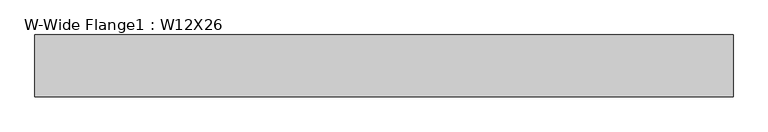
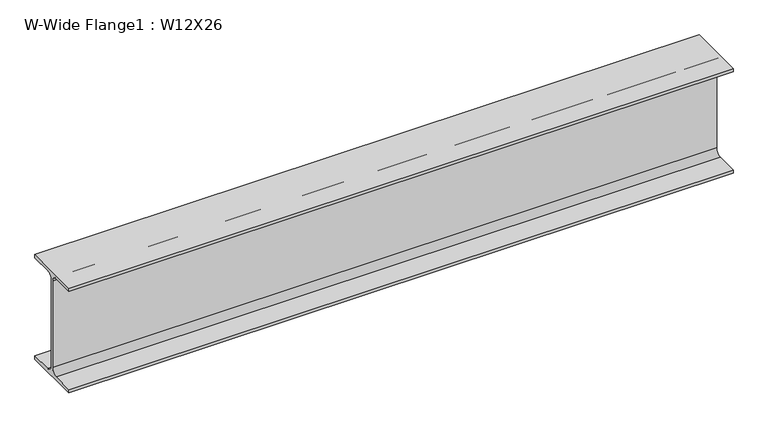
"""IFC4 building model written with IfcOpenShell, lengths in millimetres: beam geometry, W-Wide Flange1 : W12X26."""

from ifc_helpers import new_model, si_unit, point, frame, frame_2d, origin, place, context, project, spatial, polyline, circle_curve, trimmed, segment, composite_curve, outline, extrude, source, transform, mapped, element, save


def w_wide_flange1_w12x26_1be5d958(model_context):
    return source(origin(), model_context, "Body", "SweptSolid", [
        extrude(outline(composite_curve([segment(polyline([(82.423, -145.288), (82.423, -154.94), (-82.423, -154.94), (-82.423, -145.288), (-20.2565, -145.288)]), True, "CONTINUOUS"), segment(trimmed(circle_curve(frame_2d((-20.2565, -127.9525)), 17.3355), [point((-20.2565, -145.288))], [point((-2.921, -127.9525))], True, "CARTESIAN"), True, "CONTINUOUS"), segment(polyline([(-2.921, -127.9525), (-2.921, 127.9525)]), True, "CONTINUOUS"), segment(trimmed(circle_curve(frame_2d((-20.2565, 127.9525)), 17.3355), [point((-2.921, 127.9525))], [point((-20.2565, 145.288))], True, "CARTESIAN"), True, "CONTINUOUS"), segment(polyline([(-20.2565, 145.288), (-82.423, 145.288), (-82.423, 154.94), (82.423, 154.94), (82.423, 145.288), (20.2565, 145.288)]), True, "CONTINUOUS"), segment(trimmed(circle_curve(frame_2d((20.2565, 127.9525)), 17.3355), [point((20.2565, 145.288))], [point((2.921, 127.9525))], True, "CARTESIAN"), True, "CONTINUOUS"), segment(polyline([(2.921, 127.9525), (2.921, -127.9525)]), True, "CONTINUOUS"), segment(trimmed(circle_curve(frame_2d((20.2565, -127.9525)), 17.3355), [point((2.921, -127.9525))], [point((20.2565, -145.288))], True, "CARTESIAN"), True, "CONTINUOUS"), segment(polyline([(20.2565, -145.288), (82.423, -145.288)]), True, "CONTINUOUS")], self_intersect=False)), frame((-918.6128315, 0.0, 0.0), z_axis=(1.0, 0.0, 0.0), x_axis=(0.0, 1.0, 0.0)), (0.0, 0.0, 1.0), 1860.4610102),
    ])


if __name__ == "__main__":
    model = new_model("IFC4")
    model_context = context("Model", 3, world=origin())
    ifc_project = project(units=[si_unit("LENGTHUNIT", "METRE", prefix="MILLI")], contexts=[model_context])
    site = spatial("IfcSite", under=ifc_project)
    building = spatial("IfcBuilding", under=site)
    placement = place(None, origin())
    w_wide_flange1_w12x26_shape = w_wide_flange1_w12x26_1be5d958(model_context)
    element("IfcBeam", 1, ObjectType="W-Wide Flange1 : W12X26", at=placement, inside=building, context=model_context, shape_type="MappedRepresentation", body=[
        mapped(w_wide_flange1_w12x26_shape, transform((0.0, 0.0, 0.0), x_axis=(1.0, 0.0, 0.0), y_axis=(0.0, 1.0, 0.0), z_axis=(0.0, 0.0, 1.0))),
    ])
    save(model, "model.ifc")

# Revit data of these elements
# Type "W-Wide Flange1 : W12X26"
#   Assembly Code = "B10"
#   W = 26
#   Start Extension Calculation [instance default] = 10' - 0"
#   Start Extension [instance default] = -0' - 0 1/2"
#   End Extension Calculation [instance default] = 10' - 0"
#   End Extension [instance default] = -0' - 0 1/2"
#   Length [instance default] = 5' - 0"
#   bf = 0' - 6.49"
#   d = 1' - 0.2"
#   k = 0' - 1 1/16"
#   k2 = 0' - 0.6825"
#   tf = 0' - 0.38"
#   tw = 0' - 0.23"
#   A = 0.053125 SF
#   Structural Material [instance default] = Metal - Steel - ASTM A992
# Element 1 (IfcBeam, "W-Wide Flange1 : W12X26")
#   Materials on its faces: "Metal - Steel - ASTM A992"
# Materials
#   "Metal - Steel - ASTM A992": class "Metal", colour RGB 199 199 199, transparency 0
